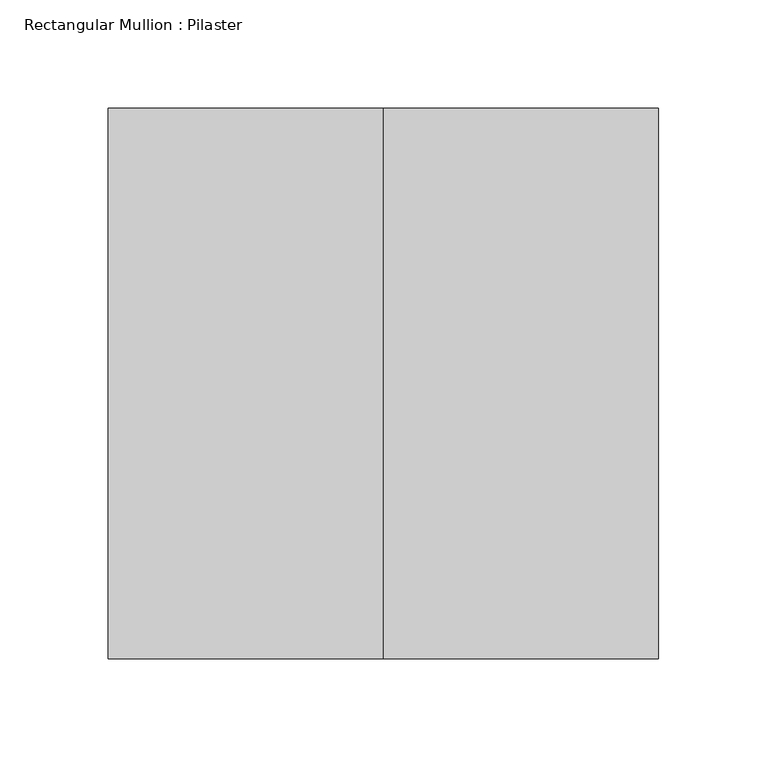
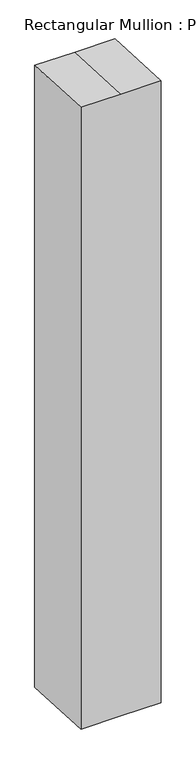
"""IFC4 building model written with IfcOpenShell, lengths in millimetres: member geometry, Rectangular Mullion : Pilaster."""

from ifc_helpers import new_model, si_unit, origin, place, context, project, spatial, faceted_brep, source, transform, mapped, element, save


def rectangular_mullion_pilaster_3233f82e(model_context):
    return source(origin(), model_context, "Body", "Brep", [
        faceted_brep([(-127.0, 127.0, -7.074079), (0.0, 127.0, -7.074079), (127.0, 127.0, -7.074079), (127.0, 127.0, -2088.7654929), (0.0, 127.0, -2088.7654929), (-127.0, 127.0, -2088.7654929), (-127.0, -127.0, 6.2374969), (-127.0, -127.0, -2075.4539169), (127.0, -127.0, 6.2374969), (0.0, -127.0, 6.2374969), (0.0, -127.0, -2075.4539169), (127.0, -127.0, -2075.4539169)], [[[0, 1, 2, 3, 4, 5]], [[6, 0, 5, 7]], [[8, 9, 6, 7, 10, 11]], [[2, 8, 11, 3]], [[2, 1, 9, 8]], [[1, 0, 6, 9]], [[3, 11, 10, 4]], [[10, 7, 5, 4]]]),
    ])


if __name__ == "__main__":
    model = new_model("IFC4")
    model_context = context("Model", 3, world=origin())
    ifc_project = project(units=[si_unit("LENGTHUNIT", "METRE", prefix="MILLI")], contexts=[model_context])
    site = spatial("IfcSite", under=ifc_project)
    building = spatial("IfcBuilding", under=site)
    placement = place(None, origin())
    rectangular_mullion_pilaster_shape = rectangular_mullion_pilaster_3233f82e(model_context)
    element("IfcMember", 1, ObjectType="Rectangular Mullion : Pilaster", at=placement, inside=building, context=model_context, shape_type="MappedRepresentation", body=[
        mapped(rectangular_mullion_pilaster_shape, transform((0.0, 0.0, 0.0), x_axis=(1.0, 0.0, 0.0), y_axis=(0.0, 1.0, 0.0), z_axis=(0.0, 0.0, 1.0))),
    ])
    save(model, "model.ifc")

# Revit data of these elements
# Type "Rectangular Mullion : Pilaster"
#   built-in parameter 1007304 = 0.833333 (stored number, unit not read)
#   built-in parameter 1007301 = 0.416667 (stored number, unit not read)
#   built-in parameter 1007300 = 0.416667 (stored number, unit not read)
# Element 1 (IfcMember, "Rectangular Mullion : Pilaster")
#   Materials on its faces: "Aluminum"
# Materials
#   "Aluminum": class "Metal", colour RGB 247 247 247, transparency 0, Description = "Aluminum 6061", Cost = 0
